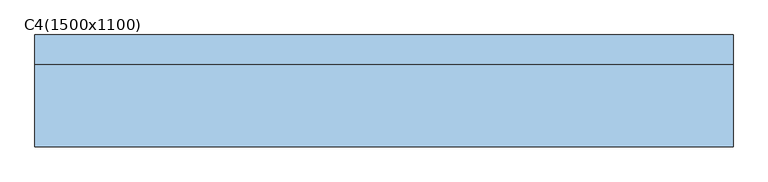
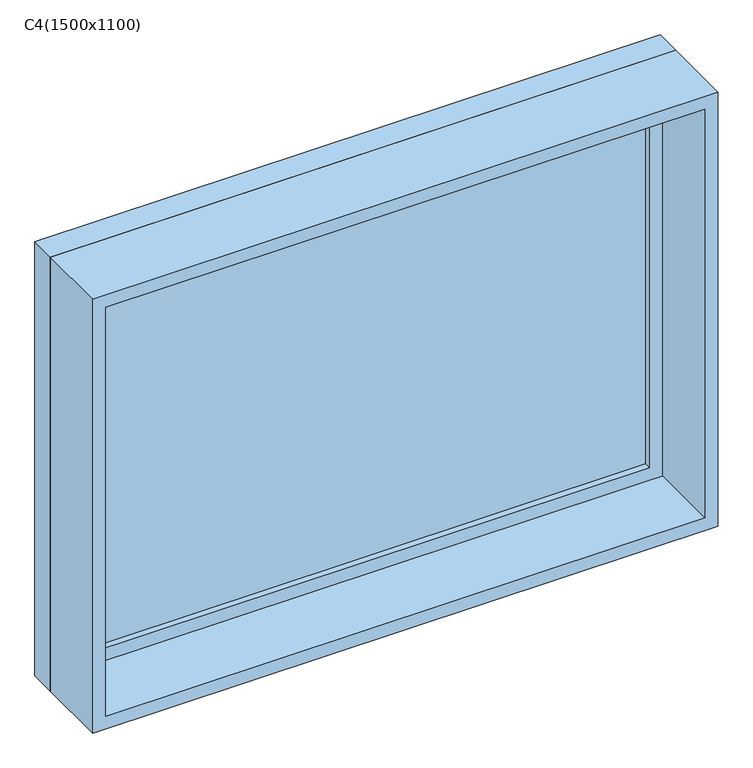
"""IFC4 building model written with IfcOpenShell, lengths in millimetres: window geometry, 固定窗 : C4(1500x1100)."""

import ifcopenshell
import ifcopenshell.guid

model = None  # the IFC model being written
_history = None  # IfcOwnerHistory: only IFC2X3 demands one
_inside = {}  # id of a spatial element -> (the spatial element, [elements in it])
_under = {}  # id of a project, library or spatial element -> (it, [spatial elements below it])
_declared = {}  # id of a project -> (the project, [libraries it declares])
_typed = {}  # id of a type object -> (the type object, [elements of that type])
_made_of = {}  # id of a material, layer set ... -> (it, [elements and type objects made of it])


def new_model(schema):
    """Start an empty IFC model of exactly this schema.

    Asked for "IFC4X3", IfcOpenShell would pick the latest addendum, in which some entities
    have other attributes; the version numbers below select the first issue.
    IFC2X3 requires an IfcOwnerHistory on every rooted entity: one is made here for all.
    """
    global model, _history
    if schema == "IFC4X3":
        model = ifcopenshell.file(schema_version=(4, 3, 0, 0))
    else:
        model = ifcopenshell.file(schema=schema)
    _inside.clear()
    _under.clear()
    _declared.clear()
    _typed.clear()
    _made_of.clear()
    _history = None
    if model.schema == "IFC2X3":
        org = make("IfcOrganization", Name="unknown")
        user = make(
            "IfcPersonAndOrganization",
            ThePerson=make("IfcPerson", FamilyName="unknown"),
            TheOrganization=org,
        )
        app = make(
            "IfcApplication",
            ApplicationDeveloper=org,
            Version="unknown",
            ApplicationFullName="unknown",
            ApplicationIdentifier="unknown",
        )
        _history = make(
            "IfcOwnerHistory",
            OwningUser=user,
            OwningApplication=app,
            ChangeAction="ADDED",
            CreationDate=0,
        )
    return model


def make(cls, **values):
    """One entity of the class cls with the attributes given. An attribute that is None is left unset."""
    return model.create_entity(
        cls, **{name: value for name, value in values.items() if value is not None}
    )


def rooted(cls, **values):
    """An entity with a GlobalId (a new one), such as an element, a storey or a relation."""
    return make(cls, GlobalId=ifcopenshell.guid.new(), OwnerHistory=_history, **values)


def si_unit(unit_type, name, prefix=None):
    """IfcSIUnit, for example si_unit("LENGTHUNIT", "METRE", prefix="MILLI")."""
    return make("IfcSIUnit", UnitType=unit_type, Prefix=prefix, Name=name)


def assignment(units):
    """IfcUnitAssignment: the units of a project."""
    return None if units is None else make("IfcUnitAssignment", Units=units)


def point(xyz):
    """IfcCartesianPoint."""
    return None if xyz is None else make("IfcCartesianPoint", Coordinates=xyz)


def direction(xyz):
    """IfcDirection."""
    return None if xyz is None else make("IfcDirection", DirectionRatios=xyz)


def frame(location, z_axis=None, x_axis=None):
    """IfcAxis2Placement3D, a coordinate frame: its origin and axes. An axis left out is left unset."""
    return make(
        "IfcAxis2Placement3D",
        Location=point(location),
        Axis=direction(z_axis),
        RefDirection=direction(x_axis),
    )


def origin():
    """The frame at (0, 0, 0) with its axes left unset."""
    return frame((0.0, 0.0, 0.0))


def place(relative_to, where):
    """IfcLocalPlacement: puts the frame where relative to a parent placement (None: the world)."""
    return make(
        "IfcLocalPlacement", PlacementRelTo=relative_to, RelativePlacement=where
    )


def context(
    kind, dimensions, precision=None, world=None, true_north=None, identifier=None
):
    """IfcGeometricRepresentationContext, for example the 3D "Model" context."""
    return make(
        "IfcGeometricRepresentationContext",
        ContextIdentifier=identifier,
        ContextType=kind,
        CoordinateSpaceDimension=dimensions,
        Precision=precision,
        WorldCoordinateSystem=world,
        TrueNorth=true_north,
    )


def project(units=None, contexts=None):
    """IfcProject with its units and contexts."""
    return rooted(
        "IfcProject",
        Name="project",
        RepresentationContexts=contexts,
        UnitsInContext=assignment(units),
    )


def spatial(cls, under=None, at=None, **own):
    """A site, building, storey or space (cls), placed at a placement, below another one or the project."""
    s = rooted(cls, ObjectPlacement=at, **own)
    if under is not None:
        _under.setdefault(under.id(), (under, []))[1].append(s)
    return s


def polyline(points):
    """IfcPolyline through the points."""
    return make("IfcPolyline", Points=[point(p) for p in points])


def outline(outer, holes=None, kind="AREA"):
    """IfcArbitraryClosedProfileDef: a profile drawn as a closed curve; with holes, ...WithVoids."""
    if holes is None:
        return make("IfcArbitraryClosedProfileDef", ProfileType=kind, OuterCurve=outer)
    return make(
        "IfcArbitraryProfileDefWithVoids",
        ProfileType=kind,
        OuterCurve=outer,
        InnerCurves=holes,
    )


def extrude(swept, where, along, depth):
    """IfcExtrudedAreaSolid: the profile swept, set in the frame where, extruded along a direction by depth."""
    return make(
        "IfcExtrudedAreaSolid",
        SweptArea=swept,
        Position=where,
        ExtrudedDirection=direction(along),
        Depth=depth,
    )


def shape(context_of_items, identifier, shape_type, items):
    """IfcShapeRepresentation: the items that make up one representation, for example the "Body"."""
    return make(
        "IfcShapeRepresentation",
        ContextOfItems=context_of_items,
        RepresentationIdentifier=identifier,
        RepresentationType=shape_type,
        Items=items,
    )


def source(mapping_origin, context_of_items, identifier, shape_type, items):
    """IfcRepresentationMap: a shape defined once, which mapped items show again and again."""
    return make(
        "IfcRepresentationMap",
        MappingOrigin=mapping_origin,
        MappedRepresentation=shape(context_of_items, identifier, shape_type, items),
    )


def transform(
    local_origin,
    x_axis=None,
    y_axis=None,
    z_axis=None,
    scale=None,
    scale2=None,
    scale3=None,
    uniform=True,
):
    """IfcCartesianTransformationOperator3D, or its non-uniform kind. x_axis, y_axis, z_axis: its Axis1, 2, 3."""
    if uniform:
        return make(
            "IfcCartesianTransformationOperator3D",
            Axis1=direction(x_axis),
            Axis2=direction(y_axis),
            LocalOrigin=point(local_origin),
            Scale=scale,
            Axis3=direction(z_axis),
        )
    return make(
        "IfcCartesianTransformationOperator3DnonUniform",
        Axis1=direction(x_axis),
        Axis2=direction(y_axis),
        LocalOrigin=point(local_origin),
        Scale=scale,
        Axis3=direction(z_axis),
        Scale2=scale2,
        Scale3=scale3,
    )


def mapped(mapping_source, mapping_target):
    """IfcMappedItem: shows the shape of a source again, moved by a transform."""
    return make(
        "IfcMappedItem", MappingSource=mapping_source, MappingTarget=mapping_target
    )


def made_of(thing, what):
    """Note that an element or type object is made of a material, layer set ...; save() writes the relation."""
    if what is not None:
        _made_of.setdefault(what.id(), (what, []))[1].append(thing)
    return thing


def element(
    cls,
    number,
    at=None,
    inside=None,
    cuts=None,
    type_object=None,
    material=None,
    context=None,
    identifier="Body",
    shape_type=None,
    held_by="IfcProductDefinitionShape",
    body=None,
    shapes=None,
    **own,
):
    """One element of the class cls, such as IfcWall. Its Tag is "e" and its number.

    at: its placement. inside: the storey or other place that contains it. cuts: it is an
    opening in that element (IfcRelVoidsElement). A single representation is given by context,
    identifier, shape_type and body (its items); several are given by shapes. held_by: the class
    of the entity that holds the representations. save() writes the other relations.
    """
    e = rooted(cls, Tag="e%d" % number, ObjectPlacement=at, **own)
    if body is not None:
        shapes = [shape(context, identifier, shape_type, body)]
    if shapes is not None:
        e.Representation = make(held_by, Representations=shapes)
    if inside is not None:
        _inside.setdefault(inside.id(), (inside, []))[1].append(e)
    if cuts is not None:
        rooted(
            "IfcRelVoidsElement", RelatingBuildingElement=cuts, RelatedOpeningElement=e
        )
    if type_object is not None:
        _typed.setdefault(type_object.id(), (type_object, []))[1].append(e)
    return made_of(e, material)


def aggregate(whole, parts):
    """IfcRelAggregates: a whole, such as a stair, and the parts it consists of."""
    return rooted("IfcRelAggregates", RelatingObject=whole, RelatedObjects=parts)


def save(model, path):
    """Write the relations noted so far, then the file.

    IfcRelAggregates (storeys below a building ...), IfcRelContainedInSpatialStructure (elements
    in a storey), IfcRelDefinesByType, IfcRelAssociatesMaterial and IfcRelDeclares: one each for
    every whole, place, type object, material and project.
    """
    for whole, parts in _under.values():
        aggregate(whole, parts)
    for where, things in _inside.values():
        rooted(
            "IfcRelContainedInSpatialStructure",
            RelatedElements=things,
            RelatingStructure=where,
        )
    for kind, things in _typed.values():
        rooted("IfcRelDefinesByType", RelatedObjects=things, RelatingType=kind)
    for what, things in _made_of.values():
        rooted("IfcRelAssociatesMaterial", RelatedObjects=things, RelatingMaterial=what)
    for by, libraries in _declared.values():
        rooted("IfcRelDeclares", RelatingContext=by, RelatedDefinitions=libraries)
    model.write(path)


def c4_1500x1100_84ff0e9f(model_context):
    return source(origin(), model_context, "Body", "SweptSolid", [
        extrude(outline(polyline([(648.4, 71.425), (-724.6, 71.425), (-724.6, 84.125), (648.4, 84.125), (648.4, 71.425)])), frame((0.0, 0.0, 963.5), z_axis=(0.0, 0.0, 1.0), x_axis=(1.0, 0.0, 0.0)), (0.0, 0.0, 1.0), 973.0),
        extrude(outline(polyline([(1980.95, -769.05), (919.05, -769.05), (919.05, 692.85), (1980.95, 692.85), (1980.95, -769.05)]), holes=[polyline([(1936.5, -724.6), (1936.5, 648.4), (963.5, 648.4), (963.5, -724.6), (1936.5, -724.6)])]), frame((0.0, 55.55, 0.0), z_axis=(0.0, 1.0, 0.0), x_axis=(0.0, 0.0, 1.0)), (0.0, 0.0, 1.0), 44.45),
        extrude(outline(polyline([(2000.0, -788.1), (900.0, -788.1), (900.0, 711.9), (2000.0, 711.9), (2000.0, -788.1)]), holes=[polyline([(1968.25, -756.35), (1968.25, 680.15), (931.75, 680.15), (931.75, -756.35), (1968.25, -756.35)])]), frame((0.0, -120.0, 0.0), z_axis=(0.0, 1.0, 0.0), x_axis=(0.0, 0.0, 1.0)), (0.0, 0.0, 1.0), 175.55),
        extrude(outline(polyline([(2000.0, 711.9), (2000.0, -788.1), (900.0, -788.1), (900.0, 711.9), (2000.0, 711.9)]), holes=[polyline([(1980.95, 692.85), (919.05, 692.85), (919.05, -769.05), (1980.95, -769.05), (1980.95, 692.85)])]), frame((0.0, 55.55, 0.0), z_axis=(0.0, 1.0, 0.0), x_axis=(0.0, 0.0, 1.0)), (0.0, 0.0, 1.0), 64.45),
    ])


if __name__ == "__main__":
    model = new_model("IFC4")
    model_context = context("Model", 3, world=origin())
    ifc_project = project(units=[si_unit("LENGTHUNIT", "METRE", prefix="MILLI")], contexts=[model_context])
    site = spatial("IfcSite", under=ifc_project)
    building = spatial("IfcBuilding", under=site)
    placement = place(None, origin())
    c4_1500x1100_shape = c4_1500x1100_84ff0e9f(model_context)
    element("IfcWindow", 1, ObjectType="固定窗 : C4(1500x1100)", at=placement, inside=building, context=model_context, shape_type="MappedRepresentation", body=[
        mapped(c4_1500x1100_shape, transform((0.0, 0.0, 0.0), x_axis=(1.0, 0.0, 0.0), y_axis=(0.0, 1.0, 0.0), z_axis=(0.0, 0.0, 1.0))),
    ])
    save(model, "model.ifc")

# Revit data of these elements
# Type "固定窗 : C4(1500x1100)"
#   Type Mark = "C1519"
#   Construction Type Id = "SGL"
#   Analytic Construction = "大型单层玻璃窗"
#   Visual Light Transmittance = 0.9
#   Solar Heat Gain Coefficient = 0.86
#   Rough Width = 1500 mm
#   Rough Height = 1100 mm
#   Heat Transfer Coefficient (U) = 5.5617 W/(m²·K)
#   Height = 1100 mm
#   默认窗台高度 = 900 mm
#   Width = 1500 mm
#   窗嵌入 = 20 mm
#   高窗平面 [instance default] = no
#   通用窗平面 [instance default] = yes
#   玻璃 = none
#   框架材质 = none
#   Wall Closure = (empty or 0)
# Element 1 (IfcWindow, "固定窗 : C4(1500x1100)")
#   Materials on its faces: "玻璃"
# Materials
#   "玻璃": class "玻璃", colour RGB 0 128 192, transparency 0.9, Description = "钠钙玻璃", Cost = 0
